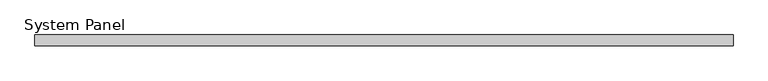
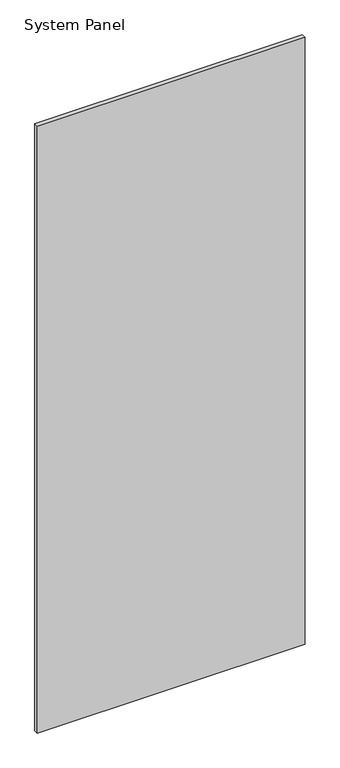
"""IFC4 building model written with IfcOpenShell, lengths in millimetres: plate geometry, System Panel : WWm-Glass-20mm-10mmOffset."""

from ifc_helpers import new_model, si_unit, origin, origin_with_axes, place, context, project, spatial, polyline, outline, extrude, source, transform, mapped, element, save


def system_panel_47cbb022(model_context):
    return source(origin(), model_context, "Body", "SweptSolid", [
        extrude(outline(polyline([(657.8305698, 0.0), (-657.8305698, 0.0), (-657.8305698, 20.0), (657.8305698, 20.0), (657.8305698, 0.0)])), origin_with_axes(), (0.0, 0.0, 1.0), 3150.0),
    ])


if __name__ == "__main__":
    model = new_model("IFC4")
    model_context = context("Model", 3, world=origin())
    ifc_project = project(units=[si_unit("LENGTHUNIT", "METRE", prefix="MILLI")], contexts=[model_context])
    site = spatial("IfcSite", under=ifc_project)
    building = spatial("IfcBuilding", under=site)
    placement = place(None, origin())
    system_panel_shape = system_panel_47cbb022(model_context)
    element("IfcPlate", 1, ObjectType="System Panel : WWm-Glass-20mm-10mmOffset", at=placement, inside=building, context=model_context, shape_type="MappedRepresentation", body=[
        mapped(system_panel_shape, transform((0.0, 0.0, 0.0), x_axis=(1.0, 0.0, 0.0), y_axis=(0.0, 1.0, 0.0), z_axis=(0.0, 0.0, 1.0))),
    ])
    save(model, "model.ifc")

# Revit data of these elements
# Type "System Panel : WWm-Glass-20mm-10mmOffset"
#   Finish = ""
# Element 1 (IfcPlate, "System Panel : WWm-Glass-20mm-10mmOffset")
#   Materials on its faces: "WW-EC-GL-Storefront"
# Materials
#   "WW-EC-GL-Storefront": class "Glass", colour RGB 236 240 239, transparency 0.85, Description = "Storefront Glass", Cost = 0
